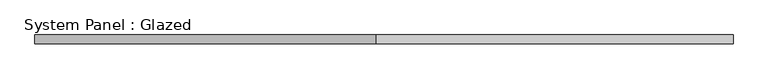
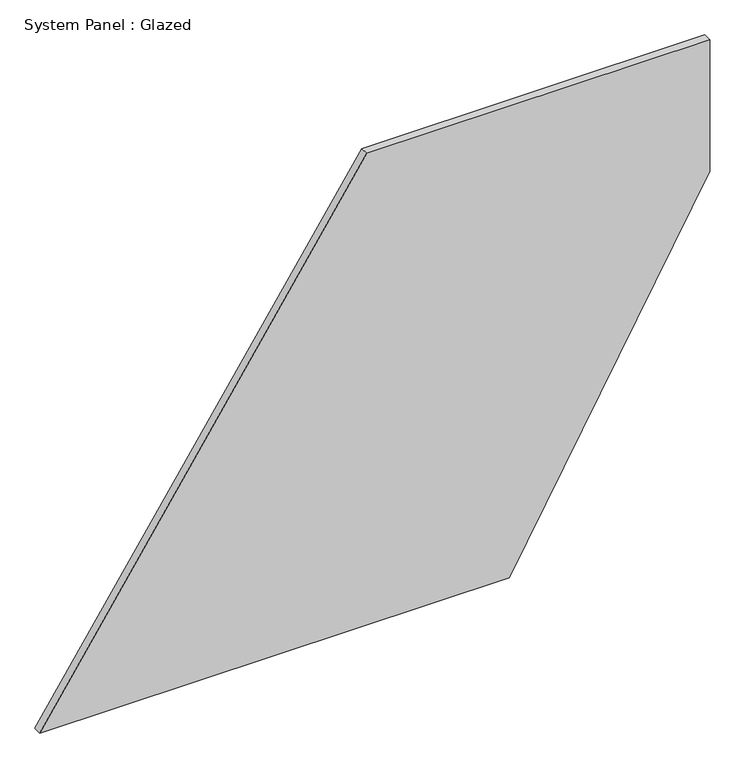
"""IFC4 building model written with IfcOpenShell, lengths in millimetres: plate geometry, System Panel : Glazed."""

from ifc_helpers import new_model, si_unit, frame, origin, place, context, project, spatial, polyline, outline, extrude, source, transform, mapped, element, save


def system_panel_glazed_a8889685(model_context):
    return source(origin(), model_context, "Body", "SweptSolid", [
        extrude(outline(polyline([(0.0, -1008.1540457), (0.0, 405.2562184), (1081.9101827, 1008.1540457), (1500.0, 1008.1540457), (1500.0, -24.4621368), (0.0, -1008.1540457)])), frame((0.0, 24.5, 0.0), z_axis=(0.0, 1.0, 0.0), x_axis=(0.0, 0.0, 1.0)), (0.0, 0.0, 1.0), 25.0),
    ])


if __name__ == "__main__":
    model = new_model("IFC4")
    model_context = context("Model", 3, world=origin())
    ifc_project = project(units=[si_unit("LENGTHUNIT", "METRE", prefix="MILLI")], contexts=[model_context])
    site = spatial("IfcSite", under=ifc_project)
    building = spatial("IfcBuilding", under=site)
    placement = place(None, origin())
    system_panel_glazed_shape = system_panel_glazed_a8889685(model_context)
    element("IfcPlate", 1, ObjectType="System Panel : Glazed", at=placement, inside=building, context=model_context, shape_type="MappedRepresentation", body=[
        mapped(system_panel_glazed_shape, transform((0.0, 0.0, 0.0), x_axis=(1.0, 0.0, 0.0), y_axis=(0.0, 1.0, 0.0), z_axis=(0.0, 0.0, 1.0))),
    ])
    save(model, "model.ifc")

# Revit data of these elements
# Type "System Panel : Glazed"
#   Construction Type Id = "GSP4R"
#   Analytic Construction = "1/8 in Pilkington single glazing"
#   Visual Light Transmittance = 0.9
#   Solar Heat Gain Coefficient = 0.86
#   Heat Transfer Coefficient (U) = 6.7069 W/(m²·K)
#   Define Thermal Properties by = 1
# Element 1 (IfcPlate, "System Panel : Glazed")
#   Materials on its faces: "Glass"
# Materials
#   "Glass": class "Glass", colour RGB 0 128 192, transparency 0.9, Description = "Soda Lime Glass", Cost = 0
